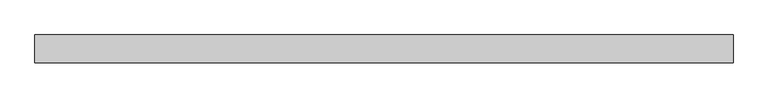
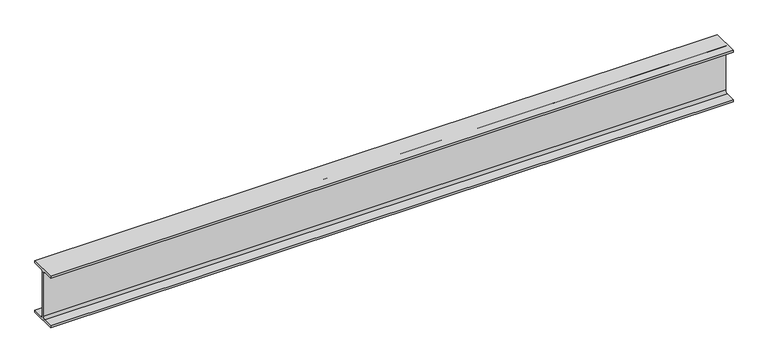
"""IFC4 building model written with IfcOpenShell, lengths in millimetres: beam geometry, 0912_Steel Framing_H-KSD3502 : H_SB_ASB_H-250x125x6x9."""

import ifcopenshell
import ifcopenshell.guid

model = None  # the IFC model being written
_history = None  # IfcOwnerHistory: only IFC2X3 demands one
_inside = {}  # id of a spatial element -> (the spatial element, [elements in it])
_under = {}  # id of a project, library or spatial element -> (it, [spatial elements below it])
_declared = {}  # id of a project -> (the project, [libraries it declares])
_typed = {}  # id of a type object -> (the type object, [elements of that type])
_made_of = {}  # id of a material, layer set ... -> (it, [elements and type objects made of it])


def new_model(schema):
    """Start an empty IFC model of exactly this schema.

    Asked for "IFC4X3", IfcOpenShell would pick the latest addendum, in which some entities
    have other attributes; the version numbers below select the first issue.
    IFC2X3 requires an IfcOwnerHistory on every rooted entity: one is made here for all.
    """
    global model, _history
    if schema == "IFC4X3":
        model = ifcopenshell.file(schema_version=(4, 3, 0, 0))
    else:
        model = ifcopenshell.file(schema=schema)
    _inside.clear()
    _under.clear()
    _declared.clear()
    _typed.clear()
    _made_of.clear()
    _history = None
    if model.schema == "IFC2X3":
        org = make("IfcOrganization", Name="unknown")
        user = make(
            "IfcPersonAndOrganization",
            ThePerson=make("IfcPerson", FamilyName="unknown"),
            TheOrganization=org,
        )
        app = make(
            "IfcApplication",
            ApplicationDeveloper=org,
            Version="unknown",
            ApplicationFullName="unknown",
            ApplicationIdentifier="unknown",
        )
        _history = make(
            "IfcOwnerHistory",
            OwningUser=user,
            OwningApplication=app,
            ChangeAction="ADDED",
            CreationDate=0,
        )
    return model


def make(cls, **values):
    """One entity of the class cls with the attributes given. An attribute that is None is left unset."""
    return model.create_entity(
        cls, **{name: value for name, value in values.items() if value is not None}
    )


def rooted(cls, **values):
    """An entity with a GlobalId (a new one), such as an element, a storey or a relation."""
    return make(cls, GlobalId=ifcopenshell.guid.new(), OwnerHistory=_history, **values)


def si_unit(unit_type, name, prefix=None):
    """IfcSIUnit, for example si_unit("LENGTHUNIT", "METRE", prefix="MILLI")."""
    return make("IfcSIUnit", UnitType=unit_type, Prefix=prefix, Name=name)


def assignment(units):
    """IfcUnitAssignment: the units of a project."""
    return None if units is None else make("IfcUnitAssignment", Units=units)


def point(xyz):
    """IfcCartesianPoint."""
    return None if xyz is None else make("IfcCartesianPoint", Coordinates=xyz)


def direction(xyz):
    """IfcDirection."""
    return None if xyz is None else make("IfcDirection", DirectionRatios=xyz)


def frame(location, z_axis=None, x_axis=None):
    """IfcAxis2Placement3D, a coordinate frame: its origin and axes. An axis left out is left unset."""
    return make(
        "IfcAxis2Placement3D",
        Location=point(location),
        Axis=direction(z_axis),
        RefDirection=direction(x_axis),
    )


def frame_2d(location, x_axis=None):
    """IfcAxis2Placement2D, a coordinate frame in the plane: its origin and x axis."""
    return make(
        "IfcAxis2Placement2D", Location=point(location), RefDirection=direction(x_axis)
    )


def origin():
    """The frame at (0, 0, 0) with its axes left unset."""
    return frame((0.0, 0.0, 0.0))


def place(relative_to, where):
    """IfcLocalPlacement: puts the frame where relative to a parent placement (None: the world)."""
    return make(
        "IfcLocalPlacement", PlacementRelTo=relative_to, RelativePlacement=where
    )


def context(
    kind, dimensions, precision=None, world=None, true_north=None, identifier=None
):
    """IfcGeometricRepresentationContext, for example the 3D "Model" context."""
    return make(
        "IfcGeometricRepresentationContext",
        ContextIdentifier=identifier,
        ContextType=kind,
        CoordinateSpaceDimension=dimensions,
        Precision=precision,
        WorldCoordinateSystem=world,
        TrueNorth=true_north,
    )


def project(units=None, contexts=None):
    """IfcProject with its units and contexts."""
    return rooted(
        "IfcProject",
        Name="project",
        RepresentationContexts=contexts,
        UnitsInContext=assignment(units),
    )


def spatial(cls, under=None, at=None, **own):
    """A site, building, storey or space (cls), placed at a placement, below another one or the project."""
    s = rooted(cls, ObjectPlacement=at, **own)
    if under is not None:
        _under.setdefault(under.id(), (under, []))[1].append(s)
    return s


def polyline(points):
    """IfcPolyline through the points."""
    return make("IfcPolyline", Points=[point(p) for p in points])


def circle_curve(where, radius):
    """IfcCircle in the frame where."""
    return make("IfcCircle", Position=where, Radius=radius)


def trimmed(basis, trim1, trim2, sense, master):
    """IfcTrimmedCurve: the piece of a basis curve between two trims."""
    return make(
        "IfcTrimmedCurve",
        BasisCurve=basis,
        Trim1=trim1,
        Trim2=trim2,
        SenseAgreement=sense,
        MasterRepresentation=master,
    )


def segment(curve, same_sense, transition):
    """IfcCompositeCurveSegment."""
    return make(
        "IfcCompositeCurveSegment",
        Transition=transition,
        SameSense=same_sense,
        ParentCurve=curve,
    )


def composite_curve(segments, self_intersect=None):
    """IfcCompositeCurve: segments joined end to end."""
    return make("IfcCompositeCurve", Segments=segments, SelfIntersect=self_intersect)


def outline(outer, holes=None, kind="AREA"):
    """IfcArbitraryClosedProfileDef: a profile drawn as a closed curve; with holes, ...WithVoids."""
    if holes is None:
        return make("IfcArbitraryClosedProfileDef", ProfileType=kind, OuterCurve=outer)
    return make(
        "IfcArbitraryProfileDefWithVoids",
        ProfileType=kind,
        OuterCurve=outer,
        InnerCurves=holes,
    )


def extrude(swept, where, along, depth):
    """IfcExtrudedAreaSolid: the profile swept, set in the frame where, extruded along a direction by depth."""
    return make(
        "IfcExtrudedAreaSolid",
        SweptArea=swept,
        Position=where,
        ExtrudedDirection=direction(along),
        Depth=depth,
    )


def shape(context_of_items, identifier, shape_type, items):
    """IfcShapeRepresentation: the items that make up one representation, for example the "Body"."""
    return make(
        "IfcShapeRepresentation",
        ContextOfItems=context_of_items,
        RepresentationIdentifier=identifier,
        RepresentationType=shape_type,
        Items=items,
    )


def source(mapping_origin, context_of_items, identifier, shape_type, items):
    """IfcRepresentationMap: a shape defined once, which mapped items show again and again."""
    return make(
        "IfcRepresentationMap",
        MappingOrigin=mapping_origin,
        MappedRepresentation=shape(context_of_items, identifier, shape_type, items),
    )


def transform(
    local_origin,
    x_axis=None,
    y_axis=None,
    z_axis=None,
    scale=None,
    scale2=None,
    scale3=None,
    uniform=True,
):
    """IfcCartesianTransformationOperator3D, or its non-uniform kind. x_axis, y_axis, z_axis: its Axis1, 2, 3."""
    if uniform:
        return make(
            "IfcCartesianTransformationOperator3D",
            Axis1=direction(x_axis),
            Axis2=direction(y_axis),
            LocalOrigin=point(local_origin),
            Scale=scale,
            Axis3=direction(z_axis),
        )
    return make(
        "IfcCartesianTransformationOperator3DnonUniform",
        Axis1=direction(x_axis),
        Axis2=direction(y_axis),
        LocalOrigin=point(local_origin),
        Scale=scale,
        Axis3=direction(z_axis),
        Scale2=scale2,
        Scale3=scale3,
    )


def mapped(mapping_source, mapping_target):
    """IfcMappedItem: shows the shape of a source again, moved by a transform."""
    return make(
        "IfcMappedItem", MappingSource=mapping_source, MappingTarget=mapping_target
    )


def made_of(thing, what):
    """Note that an element or type object is made of a material, layer set ...; save() writes the relation."""
    if what is not None:
        _made_of.setdefault(what.id(), (what, []))[1].append(thing)
    return thing


def element(
    cls,
    number,
    at=None,
    inside=None,
    cuts=None,
    type_object=None,
    material=None,
    context=None,
    identifier="Body",
    shape_type=None,
    held_by="IfcProductDefinitionShape",
    body=None,
    shapes=None,
    **own,
):
    """One element of the class cls, such as IfcWall. Its Tag is "e" and its number.

    at: its placement. inside: the storey or other place that contains it. cuts: it is an
    opening in that element (IfcRelVoidsElement). A single representation is given by context,
    identifier, shape_type and body (its items); several are given by shapes. held_by: the class
    of the entity that holds the representations. save() writes the other relations.
    """
    e = rooted(cls, Tag="e%d" % number, ObjectPlacement=at, **own)
    if body is not None:
        shapes = [shape(context, identifier, shape_type, body)]
    if shapes is not None:
        e.Representation = make(held_by, Representations=shapes)
    if inside is not None:
        _inside.setdefault(inside.id(), (inside, []))[1].append(e)
    if cuts is not None:
        rooted(
            "IfcRelVoidsElement", RelatingBuildingElement=cuts, RelatedOpeningElement=e
        )
    if type_object is not None:
        _typed.setdefault(type_object.id(), (type_object, []))[1].append(e)
    return made_of(e, material)


def aggregate(whole, parts):
    """IfcRelAggregates: a whole, such as a stair, and the parts it consists of."""
    return rooted("IfcRelAggregates", RelatingObject=whole, RelatedObjects=parts)


def save(model, path):
    """Write the relations noted so far, then the file.

    IfcRelAggregates (storeys below a building ...), IfcRelContainedInSpatialStructure (elements
    in a storey), IfcRelDefinesByType, IfcRelAssociatesMaterial and IfcRelDeclares: one each for
    every whole, place, type object, material and project.
    """
    for whole, parts in _under.values():
        aggregate(whole, parts)
    for where, things in _inside.values():
        rooted(
            "IfcRelContainedInSpatialStructure",
            RelatedElements=things,
            RelatingStructure=where,
        )
    for kind, things in _typed.values():
        rooted("IfcRelDefinesByType", RelatedObjects=things, RelatingType=kind)
    for what, things in _made_of.values():
        rooted("IfcRelAssociatesMaterial", RelatedObjects=things, RelatingMaterial=what)
    for by, libraries in _declared.values():
        rooted("IfcRelDeclares", RelatingContext=by, RelatedDefinitions=libraries)
    model.write(path)


def beam_fa849394(model_context):
    return source(origin(), model_context, "Body", "SweptSolid", [
        extrude(outline(composite_curve([segment(polyline([(62.5, -116.0), (62.5, -125.0), (-62.5, -125.0), (-62.5, -116.0), (-15.0, -116.0)]), True, "CONTINUOUS"), segment(trimmed(circle_curve(frame_2d((-15.0, -104.0)), 12.0), [point((-15.0, -116.0))], [point((-3.0, -104.0))], True, "CARTESIAN"), True, "CONTINUOUS"), segment(polyline([(-3.0, -104.0), (-3.0, 104.0)]), True, "CONTINUOUS"), segment(trimmed(circle_curve(frame_2d((-15.0, 104.0)), 12.0), [point((-3.0, 104.0))], [point((-15.0, 116.0))], True, "CARTESIAN"), True, "CONTINUOUS"), segment(polyline([(-15.0, 116.0), (-62.5, 116.0), (-62.5, 125.0), (62.5, 125.0), (62.5, 116.0), (15.0, 116.0)]), True, "CONTINUOUS"), segment(trimmed(circle_curve(frame_2d((15.0, 104.0)), 12.0), [point((15.0, 116.0))], [point((3.0, 104.0))], True, "CARTESIAN"), True, "CONTINUOUS"), segment(polyline([(3.0, 104.0), (3.0, -104.0)]), True, "CONTINUOUS"), segment(trimmed(circle_curve(frame_2d((15.0, -104.0)), 12.0), [point((3.0, -104.0))], [point((15.0, -116.0))], True, "CARTESIAN"), True, "CONTINUOUS"), segment(polyline([(15.0, -116.0), (62.5, -116.0)]), True, "CONTINUOUS")], self_intersect=False)), frame((-1494.5360727, 0.0, 0.0), z_axis=(1.0, 0.0, 0.0), x_axis=(0.0, 1.0, 0.0)), (0.0, 0.0, 1.0), 3149.3360727),
    ])


if __name__ == "__main__":
    model = new_model("IFC4")
    model_context = context("Model", 3, world=origin())
    ifc_project = project(units=[si_unit("LENGTHUNIT", "METRE", prefix="MILLI")], contexts=[model_context])
    site = spatial("IfcSite", under=ifc_project)
    building = spatial("IfcBuilding", under=site)
    placement = place(None, origin())
    beam_shape = beam_fa849394(model_context)
    element("IfcBeam", 1, ObjectType="0912_Steel Framing_H-KSD3502 : H_SB_ASB_H-250x125x6x9", at=placement, inside=building, context=model_context, shape_type="MappedRepresentation", body=[
        mapped(beam_shape, transform((0.0, 0.0, 0.0), x_axis=(1.0, 0.0, 0.0), y_axis=(0.0, 1.0, 0.0), z_axis=(0.0, 0.0, 1.0))),
    ])
    save(model, "model.ifc")

# Revit data of these elements
# Type "0912_Steel Framing_H-KSD3502 : H_SB_ASB_H-250x125x6x9"
#   H_WM Code_1 = "S01AA003-00001 | Main Steel Structure Fabrication Work | Shelter/Building | Light Steel - Standard (30KG/M>Weight) | Material: (   )"
#   H_WM Code_2 = "S03AA029-00001 | Main Steel Structure Erection Work | Shelter/Building | Light Steel (30KG/M>Weight) | Material: (   )"
#   H_WM Code_3 = "S01AA010-00001 | Main Steel Structure Fabrication Work | Shelter/Building | Steel Painting/Coating | for Non-Fireproofed Steel Surface, Surface Preparation, Primer, Second & Final Coat | Material: (   )"
#   H_Q'ty Cal Type Tag = "SB-Q2"
#   Width = 12.5 cm
#   Web Thickness = 0.6 cm
#   Web Fillet = 1.2 cm
#   Warping Constant = 42539.8 cm⁶
#   W = 0
#   Torsional Moment of Inertia = 7.8102 cm⁴
#   Section Area = 37.66 cm²
#   Plastic Modulus weak axis = 73.1 cm³
#   Plastic Modulus strong axis = 366.0 cm³
#   Perimeter = 0.97 m²/m
#   Nominal Weight = 29.60 kgf/m
#   Moment of Inertia weak axis = 294.00 cm⁴
#   Moment of Inertia strong axis = 4050.00 cm⁴
#   Height = 25.0 cm
#   Flange Thickness = 0.9 cm
#   Elastic Modulus weak axis = 47.0 cm³
#   Elastic Modulus strong axis = 324.0 cm³
#   Centroid Vertical = 12.5 cm
#   Centroid Horizontal = 6.25 cm
#   Ix = 40500000
#   Length [instance default] = 1.5240 m
#   Zx = 366000
#   b = 0.1250 m
#   h = 0.2500 m
#   r = 0.0120 m
#   s = 0.0060 m
#   t = 0.0090 m
#   A = 0.003766 m²
#   Structural Material [instance default] = Steel, 45-345
#   Assembly Code = ""
# Element 1 (IfcBeam, "0912_Steel Framing_H-KSD3502 : H_SB_ASB_H-250x125x6x9")
#   Structural Material = none
# Materials
#   "Steel, 45-345": class "Metal", colour RGB 189 187 185, transparency 0, Description = "Steel 345 MPa", Cost = 0
